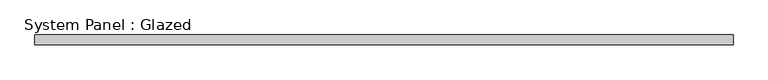
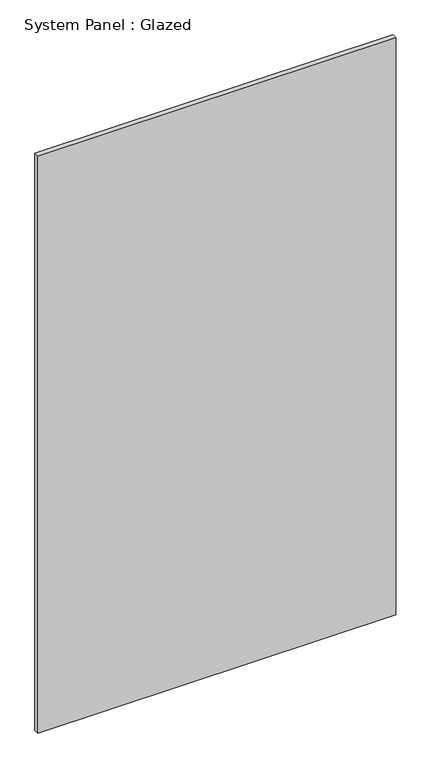
"""IFC4 building model written with IfcOpenShell, lengths in millimetres: plate geometry, System Panel : Glazed."""

from ifc_helpers import new_model, si_unit, origin, origin_with_axes, place, context, project, spatial, polyline, outline, extrude, source, transform, mapped, element, save


def system_panel_glazed_d48c6481(model_context):
    return source(origin(), model_context, "Body", "SweptSolid", [
        extrude(outline(polyline([(879.9999998, 24.5), (-879.9999998, 24.5), (-879.9999998, 49.5), (879.9999998, 49.5), (879.9999998, 24.5)])), origin_with_axes(), (0.0, 0.0, 1.0), 3000.0),
    ])


if __name__ == "__main__":
    model = new_model("IFC4")
    model_context = context("Model", 3, world=origin())
    ifc_project = project(units=[si_unit("LENGTHUNIT", "METRE", prefix="MILLI")], contexts=[model_context])
    site = spatial("IfcSite", under=ifc_project)
    building = spatial("IfcBuilding", under=site)
    placement = place(None, origin())
    system_panel_glazed_shape = system_panel_glazed_d48c6481(model_context)
    element("IfcPlate", 1, ObjectType="System Panel : Glazed", at=placement, inside=building, context=model_context, shape_type="MappedRepresentation", body=[
        mapped(system_panel_glazed_shape, transform((0.0, 0.0, 0.0), x_axis=(1.0, 0.0, 0.0), y_axis=(0.0, 1.0, 0.0), z_axis=(0.0, 0.0, 1.0))),
    ])
    save(model, "model.ifc")

# Revit data of these elements
# Type "System Panel : Glazed"
#   Construction Type Id = "GSP4R"
#   Analytic Construction = "1/8 in Pilkington single glazing"
#   Visual Light Transmittance = 0.9
#   Solar Heat Gain Coefficient = 0.86
#   Heat Transfer Coefficient (U) = 6.7069 W/(m²·K)
#   Define Thermal Properties by = 1
# Element 1 (IfcPlate, "System Panel : Glazed")
#   Materials on its faces: "Glass"
# Materials
#   "Glass": class "Glass", colour RGB 0 128 192, transparency 0.9, Description = "Soda Lime Glass", Cost = 0
